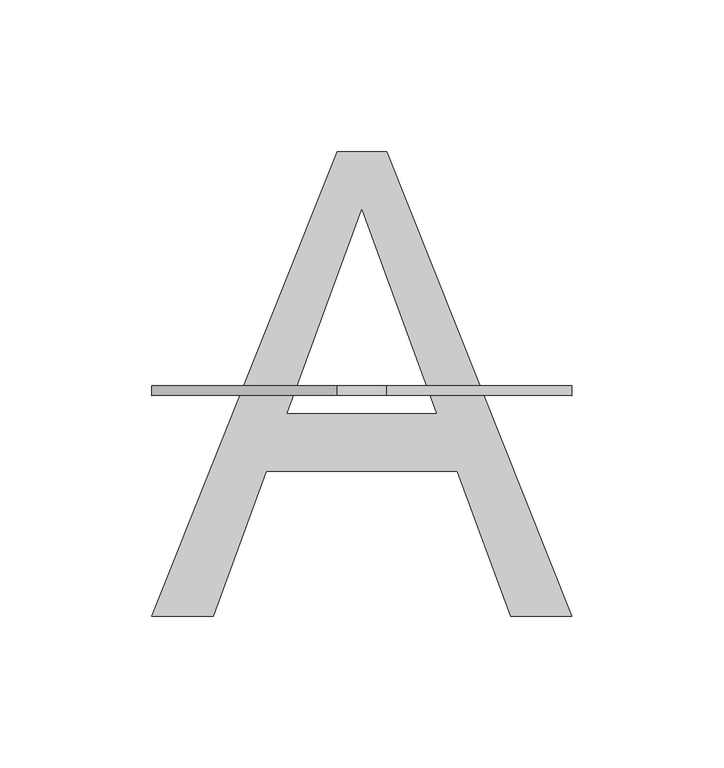
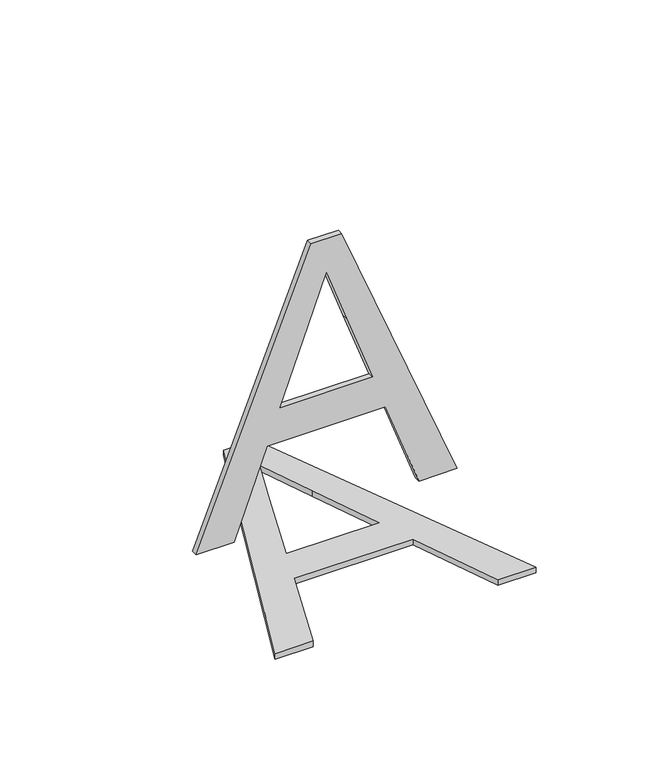
"""IFC4 building model written with IfcOpenShell, lengths in millimetres: proxy geometry, Grid Number1_FedEx : Grid Number1_FedEx."""

from ifc_helpers import new_model, si_unit, frame, origin, origin_with_axes, place, context, project, spatial, polyline, outline, extrude, source, transform, mapped, element, save


def entourage_826a01a2(model_context):
    return source(origin(), model_context, "Body", "SweptSolid", [
        extrude(outline(polyline([(-179.7252729, 146.5840649), (-118.6141874, 299.6794816), (-102.3178979, 299.6794816), (-41.2068124, 146.5840649), (-61.427667, 146.5840649), (-78.9573912, 194.4263826), (-142.0120709, 194.4263826), (-159.5044183, 146.5840649), (-179.7252729, 146.5840649)]), holes=[polyline([(-134.9852304, 213.5633097), (-85.9468548, 213.5633097), (-99.7388979, 251.2017581), (-110.4660426, 280.5425545), (-119.9971294, 254.4909174), (-134.9852304, 213.5633097)])]), origin_with_axes(), (0.0, 0.0, 1.0), 3.175),
        extrude(outline(polyline([(14.4798932, -179.7252729), (14.4798932, -159.5044183), (62.322211, -142.0120709), (62.322211, -78.9573912), (14.4798932, -61.427667), (14.4798932, -41.2068124), (167.5753099, -102.3178979), (167.5753099, -118.6141874), (14.4798932, -179.7252729)]), holes=[polyline([(81.459138, -134.9852304), (122.3867458, -119.9971294), (148.4383828, -110.4660426), (119.0975864, -99.7388979), (81.459138, -85.9468548), (81.459138, -134.9852304)])]), frame((0.0, 219.3456765, 0.0), z_axis=(0.0, 1.0, 0.0), x_axis=(0.0, 0.0, 1.0)), (0.0, 0.0, 1.0), 3.175),
    ])


if __name__ == "__main__":
    model = new_model("IFC4")
    model_context = context("Model", 3, world=origin())
    ifc_project = project(units=[si_unit("LENGTHUNIT", "METRE", prefix="MILLI")], contexts=[model_context])
    site = spatial("IfcSite", under=ifc_project)
    building = spatial("IfcBuilding", under=site)
    placement = place(None, origin())
    entourage_shape = entourage_826a01a2(model_context)
    element("IfcBuildingElementProxy", 1, Name="Grid Number1_FedEx : Grid Number1_FedEx", ObjectType="Grid Number1_FedEx : Grid Number1_FedEx", at=placement, inside=building, context=model_context, shape_type="MappedRepresentation", body=[
        mapped(entourage_shape, transform((0.0, 0.0, 0.0), x_axis=(1.0, 0.0, 0.0), y_axis=(0.0, 1.0, 0.0), z_axis=(0.0, 0.0, 1.0))),
    ])
    save(model, "model.ifc")

# Revit data of these elements
# Type "Grid Number1_FedEx : Grid Number1_FedEx"
#   Grid [instance default] = "S.8"
#   Label Width [instance default] = 1' - 0"
#   Half Box Width2 [instance default] = 0' - 6.13846"
#   Half Box Width [instance default] = 0' - 6"
#   Robust [instance default] = yes
#   Height = 0
#   Assembly Code = ""
# Element 1 (IfcBuildingElementProxy, "Grid Number1_FedEx : Grid Number1_FedEx")
#   Grid = "A"
#   Robust = no
#   Materials on its faces: "Letter"
# Materials
#   "Letter": class "Unassigned", colour RGB 178 187 30, transparency 0, Comments = "Rendering appearance not upgraded "
